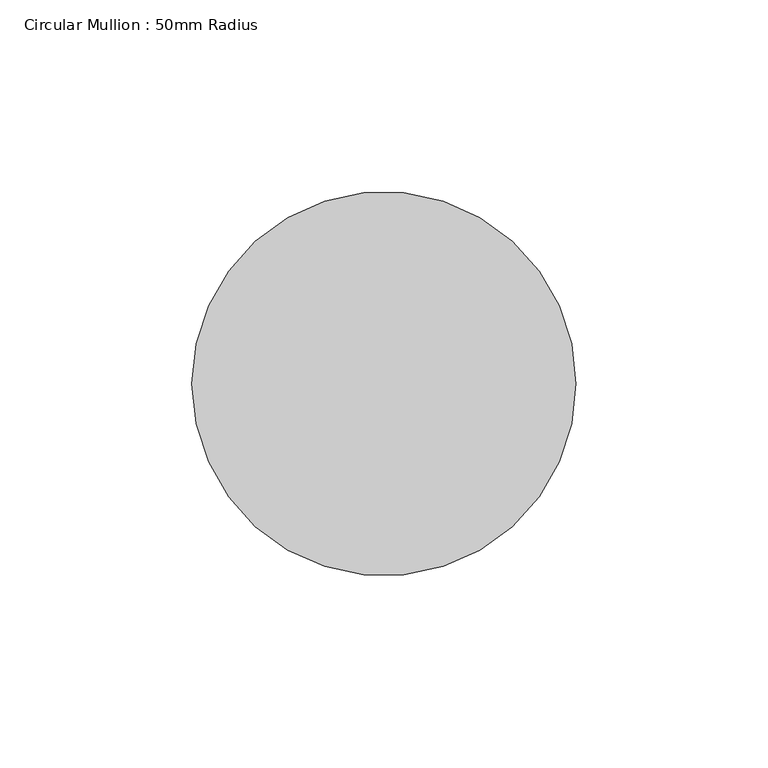
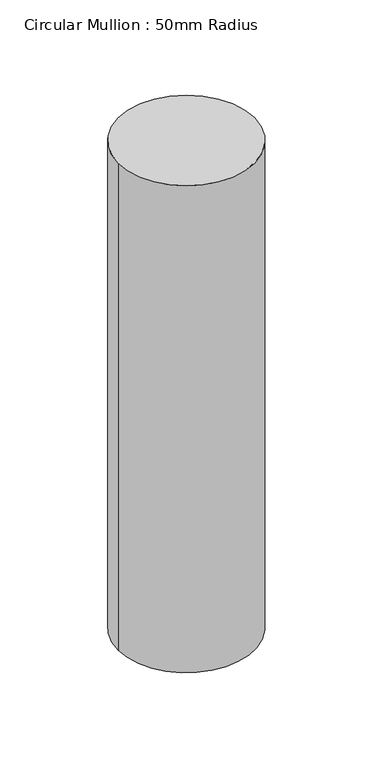
"""IFC4 building model written with IfcOpenShell, lengths in millimetres: member geometry, Circular Mullion : 50mm Radius."""

import ifcopenshell
import ifcopenshell.guid

model = None  # the IFC model being written
_history = None  # IfcOwnerHistory: only IFC2X3 demands one
_inside = {}  # id of a spatial element -> (the spatial element, [elements in it])
_under = {}  # id of a project, library or spatial element -> (it, [spatial elements below it])
_declared = {}  # id of a project -> (the project, [libraries it declares])
_typed = {}  # id of a type object -> (the type object, [elements of that type])
_made_of = {}  # id of a material, layer set ... -> (it, [elements and type objects made of it])


def new_model(schema):
    """Start an empty IFC model of exactly this schema.

    Asked for "IFC4X3", IfcOpenShell would pick the latest addendum, in which some entities
    have other attributes; the version numbers below select the first issue.
    IFC2X3 requires an IfcOwnerHistory on every rooted entity: one is made here for all.
    """
    global model, _history
    if schema == "IFC4X3":
        model = ifcopenshell.file(schema_version=(4, 3, 0, 0))
    else:
        model = ifcopenshell.file(schema=schema)
    _inside.clear()
    _under.clear()
    _declared.clear()
    _typed.clear()
    _made_of.clear()
    _history = None
    if model.schema == "IFC2X3":
        org = make("IfcOrganization", Name="unknown")
        user = make(
            "IfcPersonAndOrganization",
            ThePerson=make("IfcPerson", FamilyName="unknown"),
            TheOrganization=org,
        )
        app = make(
            "IfcApplication",
            ApplicationDeveloper=org,
            Version="unknown",
            ApplicationFullName="unknown",
            ApplicationIdentifier="unknown",
        )
        _history = make(
            "IfcOwnerHistory",
            OwningUser=user,
            OwningApplication=app,
            ChangeAction="ADDED",
            CreationDate=0,
        )
    return model


def make(cls, **values):
    """One entity of the class cls with the attributes given. An attribute that is None is left unset."""
    return model.create_entity(
        cls, **{name: value for name, value in values.items() if value is not None}
    )


def rooted(cls, **values):
    """An entity with a GlobalId (a new one), such as an element, a storey or a relation."""
    return make(cls, GlobalId=ifcopenshell.guid.new(), OwnerHistory=_history, **values)


def si_unit(unit_type, name, prefix=None):
    """IfcSIUnit, for example si_unit("LENGTHUNIT", "METRE", prefix="MILLI")."""
    return make("IfcSIUnit", UnitType=unit_type, Prefix=prefix, Name=name)


def assignment(units):
    """IfcUnitAssignment: the units of a project."""
    return None if units is None else make("IfcUnitAssignment", Units=units)


def point(xyz):
    """IfcCartesianPoint."""
    return None if xyz is None else make("IfcCartesianPoint", Coordinates=xyz)


def direction(xyz):
    """IfcDirection."""
    return None if xyz is None else make("IfcDirection", DirectionRatios=xyz)


def frame(location, z_axis=None, x_axis=None):
    """IfcAxis2Placement3D, a coordinate frame: its origin and axes. An axis left out is left unset."""
    return make(
        "IfcAxis2Placement3D",
        Location=point(location),
        Axis=direction(z_axis),
        RefDirection=direction(x_axis),
    )


def frame_2d(location, x_axis=None):
    """IfcAxis2Placement2D, a coordinate frame in the plane: its origin and x axis."""
    return make(
        "IfcAxis2Placement2D", Location=point(location), RefDirection=direction(x_axis)
    )


def origin():
    """The frame at (0, 0, 0) with its axes left unset."""
    return frame((0.0, 0.0, 0.0))


def origin_2d():
    """The frame at (0, 0) in the plane with its x axis left unset."""
    return frame_2d((0.0, 0.0))


def place(relative_to, where):
    """IfcLocalPlacement: puts the frame where relative to a parent placement (None: the world)."""
    return make(
        "IfcLocalPlacement", PlacementRelTo=relative_to, RelativePlacement=where
    )


def context(
    kind, dimensions, precision=None, world=None, true_north=None, identifier=None
):
    """IfcGeometricRepresentationContext, for example the 3D "Model" context."""
    return make(
        "IfcGeometricRepresentationContext",
        ContextIdentifier=identifier,
        ContextType=kind,
        CoordinateSpaceDimension=dimensions,
        Precision=precision,
        WorldCoordinateSystem=world,
        TrueNorth=true_north,
    )


def project(units=None, contexts=None):
    """IfcProject with its units and contexts."""
    return rooted(
        "IfcProject",
        Name="project",
        RepresentationContexts=contexts,
        UnitsInContext=assignment(units),
    )


def spatial(cls, under=None, at=None, **own):
    """A site, building, storey or space (cls), placed at a placement, below another one or the project."""
    s = rooted(cls, ObjectPlacement=at, **own)
    if under is not None:
        _under.setdefault(under.id(), (under, []))[1].append(s)
    return s


def circle_curve(where, radius):
    """IfcCircle in the frame where."""
    return make("IfcCircle", Position=where, Radius=radius)


def trimmed(basis, trim1, trim2, sense, master):
    """IfcTrimmedCurve: the piece of a basis curve between two trims."""
    return make(
        "IfcTrimmedCurve",
        BasisCurve=basis,
        Trim1=trim1,
        Trim2=trim2,
        SenseAgreement=sense,
        MasterRepresentation=master,
    )


def segment(curve, same_sense, transition):
    """IfcCompositeCurveSegment."""
    return make(
        "IfcCompositeCurveSegment",
        Transition=transition,
        SameSense=same_sense,
        ParentCurve=curve,
    )


def composite_curve(segments, self_intersect=None):
    """IfcCompositeCurve: segments joined end to end."""
    return make("IfcCompositeCurve", Segments=segments, SelfIntersect=self_intersect)


def outline(outer, holes=None, kind="AREA"):
    """IfcArbitraryClosedProfileDef: a profile drawn as a closed curve; with holes, ...WithVoids."""
    if holes is None:
        return make("IfcArbitraryClosedProfileDef", ProfileType=kind, OuterCurve=outer)
    return make(
        "IfcArbitraryProfileDefWithVoids",
        ProfileType=kind,
        OuterCurve=outer,
        InnerCurves=holes,
    )


def extrude(swept, where, along, depth):
    """IfcExtrudedAreaSolid: the profile swept, set in the frame where, extruded along a direction by depth."""
    return make(
        "IfcExtrudedAreaSolid",
        SweptArea=swept,
        Position=where,
        ExtrudedDirection=direction(along),
        Depth=depth,
    )


def shape(context_of_items, identifier, shape_type, items):
    """IfcShapeRepresentation: the items that make up one representation, for example the "Body"."""
    return make(
        "IfcShapeRepresentation",
        ContextOfItems=context_of_items,
        RepresentationIdentifier=identifier,
        RepresentationType=shape_type,
        Items=items,
    )


def source(mapping_origin, context_of_items, identifier, shape_type, items):
    """IfcRepresentationMap: a shape defined once, which mapped items show again and again."""
    return make(
        "IfcRepresentationMap",
        MappingOrigin=mapping_origin,
        MappedRepresentation=shape(context_of_items, identifier, shape_type, items),
    )


def transform(
    local_origin,
    x_axis=None,
    y_axis=None,
    z_axis=None,
    scale=None,
    scale2=None,
    scale3=None,
    uniform=True,
):
    """IfcCartesianTransformationOperator3D, or its non-uniform kind. x_axis, y_axis, z_axis: its Axis1, 2, 3."""
    if uniform:
        return make(
            "IfcCartesianTransformationOperator3D",
            Axis1=direction(x_axis),
            Axis2=direction(y_axis),
            LocalOrigin=point(local_origin),
            Scale=scale,
            Axis3=direction(z_axis),
        )
    return make(
        "IfcCartesianTransformationOperator3DnonUniform",
        Axis1=direction(x_axis),
        Axis2=direction(y_axis),
        LocalOrigin=point(local_origin),
        Scale=scale,
        Axis3=direction(z_axis),
        Scale2=scale2,
        Scale3=scale3,
    )


def mapped(mapping_source, mapping_target):
    """IfcMappedItem: shows the shape of a source again, moved by a transform."""
    return make(
        "IfcMappedItem", MappingSource=mapping_source, MappingTarget=mapping_target
    )


def made_of(thing, what):
    """Note that an element or type object is made of a material, layer set ...; save() writes the relation."""
    if what is not None:
        _made_of.setdefault(what.id(), (what, []))[1].append(thing)
    return thing


def element(
    cls,
    number,
    at=None,
    inside=None,
    cuts=None,
    type_object=None,
    material=None,
    context=None,
    identifier="Body",
    shape_type=None,
    held_by="IfcProductDefinitionShape",
    body=None,
    shapes=None,
    **own,
):
    """One element of the class cls, such as IfcWall. Its Tag is "e" and its number.

    at: its placement. inside: the storey or other place that contains it. cuts: it is an
    opening in that element (IfcRelVoidsElement). A single representation is given by context,
    identifier, shape_type and body (its items); several are given by shapes. held_by: the class
    of the entity that holds the representations. save() writes the other relations.
    """
    e = rooted(cls, Tag="e%d" % number, ObjectPlacement=at, **own)
    if body is not None:
        shapes = [shape(context, identifier, shape_type, body)]
    if shapes is not None:
        e.Representation = make(held_by, Representations=shapes)
    if inside is not None:
        _inside.setdefault(inside.id(), (inside, []))[1].append(e)
    if cuts is not None:
        rooted(
            "IfcRelVoidsElement", RelatingBuildingElement=cuts, RelatedOpeningElement=e
        )
    if type_object is not None:
        _typed.setdefault(type_object.id(), (type_object, []))[1].append(e)
    return made_of(e, material)


def aggregate(whole, parts):
    """IfcRelAggregates: a whole, such as a stair, and the parts it consists of."""
    return rooted("IfcRelAggregates", RelatingObject=whole, RelatedObjects=parts)


def save(model, path):
    """Write the relations noted so far, then the file.

    IfcRelAggregates (storeys below a building ...), IfcRelContainedInSpatialStructure (elements
    in a storey), IfcRelDefinesByType, IfcRelAssociatesMaterial and IfcRelDeclares: one each for
    every whole, place, type object, material and project.
    """
    for whole, parts in _under.values():
        aggregate(whole, parts)
    for where, things in _inside.values():
        rooted(
            "IfcRelContainedInSpatialStructure",
            RelatedElements=things,
            RelatingStructure=where,
        )
    for kind, things in _typed.values():
        rooted("IfcRelDefinesByType", RelatedObjects=things, RelatingType=kind)
    for what, things in _made_of.values():
        rooted("IfcRelAssociatesMaterial", RelatedObjects=things, RelatingMaterial=what)
    for by, libraries in _declared.values():
        rooted("IfcRelDeclares", RelatingContext=by, RelatedDefinitions=libraries)
    model.write(path)


def circular_mullion_50mm_radius_97ae94e2(model_context):
    return source(origin(), model_context, "Body", "SweptSolid", [
        extrude(outline(composite_curve([segment(trimmed(circle_curve(origin_2d(), 50.0), [point((50.0, 0.0))], [point((-50.0, 0.0))], False, "CARTESIAN"), True, "CONTINUOUS"), segment(trimmed(circle_curve(origin_2d(), 50.0), [point((-50.0, 0.0))], [point((50.0, 0.0))], False, "CARTESIAN"), True, "CONTINUOUS")], self_intersect=False)), frame((0.0, 0.0, -377.4891476), z_axis=(0.0, 0.0, 1.0), x_axis=(1.0, 0.0, 0.0)), (0.0, 0.0, 1.0), 377.4891476),
    ])


if __name__ == "__main__":
    model = new_model("IFC4")
    model_context = context("Model", 3, world=origin())
    ifc_project = project(units=[si_unit("LENGTHUNIT", "METRE", prefix="MILLI")], contexts=[model_context])
    site = spatial("IfcSite", under=ifc_project)
    building = spatial("IfcBuilding", under=site)
    placement = place(None, origin())
    circular_mullion_50mm_radius_shape = circular_mullion_50mm_radius_97ae94e2(model_context)
    element("IfcMember", 1, ObjectType="Circular Mullion : 50mm Radius", at=placement, inside=building, context=model_context, shape_type="MappedRepresentation", body=[
        mapped(circular_mullion_50mm_radius_shape, transform((0.0, 0.0, 0.0), x_axis=(1.0, 0.0, 0.0), y_axis=(0.0, 1.0, 0.0), z_axis=(0.0, 0.0, 1.0))),
    ])
    save(model, "model.ifc")

# Revit data of these elements
# Type "Circular Mullion : 50mm Radius"
#   built-in parameter 1007350 = 0.164042 (stored number, unit not read)
# Element 1 (IfcMember, "Circular Mullion : 50mm Radius")
#   Materials on its faces: "Aluminium"
# Materials
#   "Aluminium": class "Metal", colour RGB 247 247 247, transparency 0, Description = "Aluminium 6061", Cost = 0
